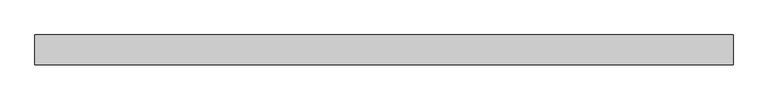
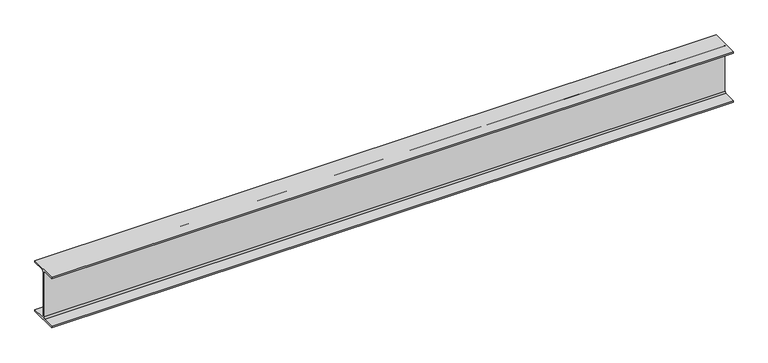
"""IFC4 building model written with IfcOpenShell, lengths in millimetres: beam geometry, Old_Steel Beam_H-KSD3502 : H_SB_ASB_H-250×125x6x9."""

from ifc_helpers import new_model, si_unit, point, frame, frame_2d, origin, place, context, project, spatial, polyline, circle_curve, trimmed, segment, composite_curve, outline, extrude, source, transform, mapped, element, save


def beam_197d14ed(model_context):
    return source(origin(), model_context, "Body", "SweptSolid", [
        extrude(outline(composite_curve([segment(polyline([(82.5, -141.5), (82.5, -151.7), (-82.5, -151.7), (-82.5, -141.5), (-11.9, -141.5)]), True, "CONTINUOUS"), segment(trimmed(circle_curve(frame_2d((-11.9, -132.6)), 8.9), [point((-11.9, -141.5))], [point((-3.0, -132.6))], True, "CARTESIAN"), True, "CONTINUOUS"), segment(polyline([(-3.0, -132.6), (-3.0, 132.6)]), True, "CONTINUOUS"), segment(trimmed(circle_curve(frame_2d((-11.9, 132.6)), 8.9), [point((-3.0, 132.6))], [point((-11.9, 141.5))], True, "CARTESIAN"), True, "CONTINUOUS"), segment(polyline([(-11.9, 141.5), (-82.5, 141.5), (-82.5, 151.7), (82.5, 151.7), (82.5, 141.5), (11.9, 141.5)]), True, "CONTINUOUS"), segment(trimmed(circle_curve(frame_2d((11.9, 132.6)), 8.9), [point((11.9, 141.5))], [point((3.0, 132.6))], True, "CARTESIAN"), True, "CONTINUOUS"), segment(polyline([(3.0, 132.6), (3.0, -132.6)]), True, "CONTINUOUS"), segment(trimmed(circle_curve(frame_2d((11.9, -132.6)), 8.9), [point((3.0, -132.6))], [point((11.9, -141.5))], True, "CARTESIAN"), True, "CONTINUOUS"), segment(polyline([(11.9, -141.5), (82.5, -141.5)]), True, "CONTINUOUS")], self_intersect=False)), frame((-2029.8, 0.0, 0.0), z_axis=(1.0, 0.0, 0.0), x_axis=(0.0, 1.0, 0.0)), (0.0, 0.0, 1.0), 3859.8827532),
    ])


if __name__ == "__main__":
    model = new_model("IFC4")
    model_context = context("Model", 3, world=origin())
    ifc_project = project(units=[si_unit("LENGTHUNIT", "METRE", prefix="MILLI")], contexts=[model_context])
    site = spatial("IfcSite", under=ifc_project)
    building = spatial("IfcBuilding", under=site)
    placement = place(None, origin())
    beam_shape = beam_197d14ed(model_context)
    element("IfcBeam", 1, ObjectType="Old_Steel Beam_H-KSD3502 : H_SB_ASB_H-250×125x6x9", at=placement, inside=building, context=model_context, shape_type="MappedRepresentation", body=[
        mapped(beam_shape, transform((0.0, 0.0, 0.0), x_axis=(1.0, 0.0, 0.0), y_axis=(0.0, 1.0, 0.0), z_axis=(0.0, 0.0, 1.0))),
    ])
    save(model, "model.ifc")

# Revit data of these elements
# Type "Old_Steel Beam_H-KSD3502 : H_SB_ASB_H-250×125x6x9"
#   Width = 12.5 cm
#   Web Thickness = 0.6 cm
#   Web Fillet = 1.2 cm
#   Warping Constant = 42539.8 cm⁶
#   Torsional Moment of Inertia = 7.8102 cm⁴
#   Torsional Modulus = 1.0 cm³
#   Section Area = 37.66 cm²
#   Plastic Modulus weak axis = 73.1 cm³
#   Plastic Modulus strong axis = 366.0 cm³
#   Perimeter = 0.97 m²/m
#   Nominal Weight = 29.60 kgf/m
#   Moment of Inertia weak axis = 294.00 cm⁴
#   Moment of Inertia strong axis = 4050.00 cm⁴
#   Height = 25.0 cm
#   Flange Thickness = 0.9 cm
#   Elastic Modulus weak axis = 47.0 cm³
#   Elastic Modulus strong axis = 324.0 cm³
#   Centroid Vertical = 12.5 cm
#   Centroid Horizontal = 6.25 cm
#   Length [instance default] = 1.5240 m
#   Structural Material [instance default] = Steel, 45-345
#   Assembly Code = ""
# Element 1 (IfcBeam, "Old_Steel Beam_H-KSD3502 : H_SB_ASB_H-250×125x6x9")
#   Structural Material = none
# Materials
#   "Steel, 45-345": class "Metal", colour RGB 189 187 185, transparency 0, Description = "Steel 345 MPa", Cost = 0
